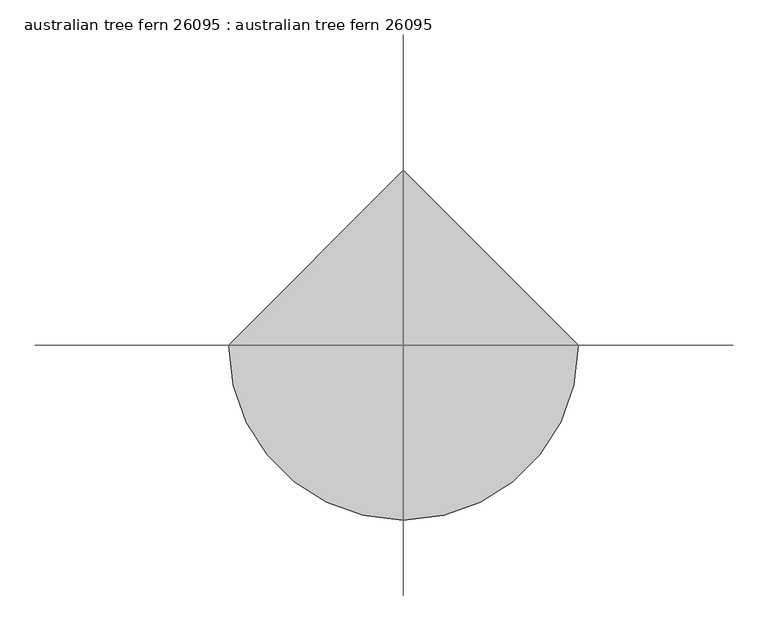
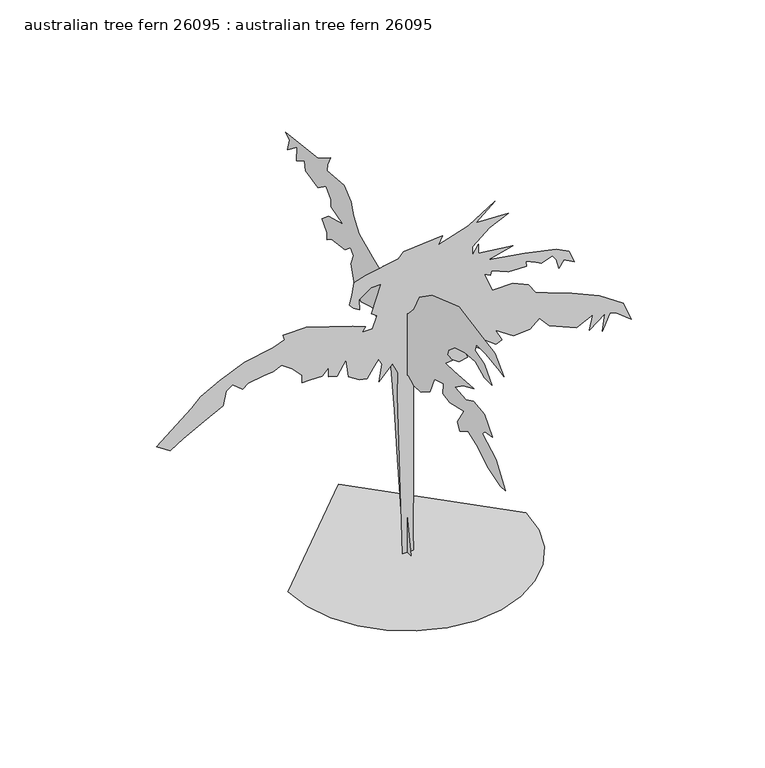
"""IFC4 building model written with IfcOpenShell, lengths in millimetres: proxy geometry, australian tree fern 26095 : australian tree fern 26095."""

from ifc_helpers import new_model, si_unit, origin, place, context, project, spatial, triangles, source, transform, mapped, element, save


def australian_tree_fern_26095_australian_tree_fern_26095_77f1a640(model_context):
    return source(origin(), model_context, "Body", "Tessellation", [
        triangles([(-639.0365753, 0.0, 0.0007159), (-622.1405136, -146.4247652, 0.0007159), (-574.0277527, -280.8912123, 0.0007159), (-498.5465315, -399.5499215, 0.0007159), (-399.5499215, -498.5465315, 0.0007159), (-280.8912123, -574.0277527, 0.0007159), (-146.4247652, -622.1405136, 0.0007159), (2.79e-05, -639.0365753, 0.0007159), (146.4247652, -622.1429844, 0.0007159), (280.8912123, -574.0277527, 0.0007159), (399.5499215, -498.5465315, 0.0007159), (498.5465315, -399.5499215, 0.0007159), (574.0277527, -280.8912123, 0.0007159), (622.1405136, -146.4247652, 0.0007159), (639.0365753, 5.59e-05, 0.0007159), (-8.38e-05, 639.0365753, 0.0007159), (470.2991641, -3.5e-05, 1828.8014534), (368.5593713, -2.98e-05, 1741.5955845), (542.9711454, -2.94e-05, 1734.3285862), (441.231389, -2.66e-05, 1687.0922253), (350.3907492, -2.2e-05, 1610.7880165), (350.3907492, -1.92e-05, 1563.5516556), (383.0932589, -2.22e-05, 1614.4202076), (383.0932589, -1.92e-05, 1563.5516556), (568.4067295, -1.79e-05, 1541.750806), (437.5966181, -1.59e-05, 1509.0482964), (633.8092781, -1.4e-05, 1476.3456413), (800.9540903, -1.18e-05, 1440.0109406), (869.9913008, -9.7e-06, 1403.673769), (899.0591486, -5.5e-06, 1334.6364132), (840.9235256, -7.5e-06, 1367.3389229), (815.4879416, -5.1e-06, 1327.3695602), (800.9540903, -8.4e-06, 1381.8729195), (779.1532408, -1.01e-05, 1410.9406219), (721.015147, -8.8e-06, 1389.1397724), (691.9473719, -9.7e-06, 1403.673769), (637.4440126, -1.12e-05, 1429.1092804), (641.0762037, -9.4e-06, 1400.0414326), (597.4745047, -9.4e-06, 1400.0414326), (542.9711454, -9.7e-06, 1403.673769), (452.1330491, -1.18e-05, 1440.0109406), (448.4983146, -1.03e-05, 1414.5754292), (415.7958049, -1.14e-05, 1432.7440876), (459.4000111, -5.1e-06, 1327.3695602), (568.4067295, -5.1e-06, 1327.3695602), (651.9778639, -2.9e-06, 1291.0347141), (688.3126373, 3e-07, 1236.5313549), (753.7176567, 1.8e-06, 1211.0958435), (884.5252247, 4.9e-06, 1160.2246754), (1033.5014511, 8.7e-06, 1094.8221268), (1160.6767553, 1.39e-05, 1007.6162579), (1204.2784544, 2.02e-05, 902.2417305), (1120.70732, 1.63e-05, 967.6468225), (1088.0048103, 1.59e-05, 974.9137482), (1048.0353024, 2.11e-05, 887.7078793), (1062.5692263, 1.55e-05, 982.1806738), (978.9980919, 1.94e-05, 916.7781979), (997.1666777, 1.44e-05, 1000.3493322), (909.9608088, 1.7e-05, 956.7450897), (764.6193169, 1.33e-05, 1018.5179907), (710.1159576, 9.6e-06, 1080.2882755), (659.2448622, 1.22e-05, 1036.684033), (572.0389206, 1.26e-05, 1029.4171074), (473.9338986, 8.7e-06, 1094.8221268), (510.2686357, 1.26e-05, 1029.4171074), (477.5660897, 1.35e-05, 1014.8831835), (324.9577085, 6.6e-06, 1131.1569002), (419.4305394, 1.44e-05, 1000.3493322), (284.9882369, 8.7e-06, 1094.8221268), (324.9577085, 1.48e-05, 993.0824066), (277.7212749, 1.52e-05, 985.8154083), (190.5151335, 1.16e-05, 1047.5857658), (88.7756132, 9.6e-06, 1080.2882755), (194.1488688, 1.52e-05, 985.8154083), (30.6385209, 1.11e-05, 1054.8526915), (34.2719928, 1.57e-05, 978.5484827), (34.2719928, 3.32e-05, 684.2282936), (34.2719928, 4.84e-05, 429.8801196), (30.6385209, 6.77e-05, 106.4923825), (34.2719928, 7.35e-05, 0.0013276), (-23.8650472, 7.39e-05, 0.0007003), (-52.9336422, 1.98e-05, 909.5111996), (-49.2999159, 1.22e-05, 1036.684033), (-78.3684632, 8.5e-06, 1098.4543905), (-151.0396997, 1.31e-05, 1022.1501818), (-136.5055487, 7.5e-06, 1116.6229763), (-154.6734259, 5.5e-06, 1149.325486), (-183.7417098, 7.9e-06, 1109.3560507), (-216.4437289, 1.07e-05, 1062.1196171), (-256.4132006, 1.03e-05, 1069.3865427), (-314.5512943, 8.1e-06, 1105.7213161), (-329.0852182, 2e-06, 1207.461109), (-376.3216155, 6.6e-06, 1131.1569002), (-423.5580491, 5.7e-06, 1145.6907515), (-423.5580491, 2.7e-06, 1196.5619196), (-456.2580153, 4.9e-06, 1160.2246754), (-518.0283365, 4.9e-06, 1160.2246754), (-565.2647701, 4.9e-06, 1160.2246754), (-565.2647701, 2.3e-06, 1203.8289179), (-619.7706728, -1e-06, 1258.3322044), (-674.2714886, -3.4e-06, 1298.3017124), (-721.5079222, -2.1e-06, 1276.5008629), (-772.3790903, -1.9e-06, 1272.866201), (-855.9502247, -1e-06, 1258.3322044), (-885.0205433, 3e-07, 1236.5313549), (-939.5239025, -2.3e-06, 1280.133054), (-972.2238688, -8e-07, 1254.6975426), (-990.3925272, 3.8e-06, 1178.3933338), (-1092.13232, 6.8e-06, 1127.5247091), (-1204.773773, 1.05e-05, 1065.7543516), (-1273.8110561, 1.31e-05, 1022.1501818), (-1346.4830738, 1.03e-05, 1069.3865427), (-1157.5373394, 1.2e-06, 1221.9975037), (-1110.3009058, -1.9e-06, 1272.866201), (-1008.561113, -5.1e-06, 1327.3695602), (-874.1188105, -8.6e-06, 1385.5075813), (-721.5079222, -1.03e-05, 1414.5754292), (-659.7375647, -1.16e-05, 1436.3762787), (-667.004563, -1.33e-05, 1465.4439812), (-539.8317295, -1.33e-05, 1465.4439812), (-416.2885437, -1.1e-05, 1425.4770893), (-292.7479377, -8.6e-06, 1385.5075813), (-223.7109271, -7.1e-06, 1360.0720699), (-241.8788043, -5.5e-06, 1334.6364132), (-187.3751907, -5.5e-06, 1334.6364132), (-161.9403697, -9.4e-06, 1400.0414326), (-191.0089079, -1.07e-05, 1421.8422821), (-140.1390206, -1.96e-05, 1570.8185085), (-194.6423889, -1.96e-05, 1570.8185085), (-260.0454098, -1.68e-05, 1523.5821476), (-256.4132006, -1.33e-05, 1465.4439812), (-289.1157284, -1.46e-05, 1487.2474468), (-310.9165598, -1.62e-05, 1512.6804874), (-296.3826722, -1.94e-05, 1567.1838467), (-285.4809939, -2.31e-05, 1628.956675), (-220.0774642, -2.44e-05, 1650.7575245), (-45.666444, -2.63e-05, 1683.4600342), (-20.2313959, -2.81e-05, 1712.5277367), (190.5151335, -2.92e-05, 1730.6963951), (168.7137935, -2.66e-05, 1687.0922253), (328.5898996, -2.96e-05, 1737.9633934), (3.03e-05, -861.8582216, 1549.8330162), (2.4e-05, -733.5424347, 1570.5289913), (2.01e-05, -646.6209961, 1570.5289913), (2.06e-05, -630.0627771, 1529.1370411), (2.54e-05, -721.12437, 1504.3009117), (3.07e-05, -787.3523769, 1425.6574562), (2.76e-05, -716.9866865, 1425.6574562), (2.26e-05, -634.2029314, 1467.0492611), (1.86e-05, -539.0011479, 1458.7689526), (1.52e-05, -443.8018716, 1429.7951397), (1.41e-05, -385.8542459, 1380.1253517), (1.46e-05, -373.4361812, 1347.0113846), (1.68e-05, -423.1059328, 1347.0113846), (1.55e-05, -356.8778895, 1289.0637589), (1.89e-05, -435.5239975, 1293.2039131), (2.69e-05, -621.7848667, 1305.6220505), (2.36e-05, -518.3052092, 1260.089946), (2.19e-05, -443.8018716, 1206.2800037), (2.68e-05, -547.2815291, 1198.0020933), (2.89e-05, -617.6471832, 1231.1161331), (3.37e-05, -716.9866865, 1218.6980684), (3.97e-05, -795.6302147, 1135.9143133), (3.69e-05, -725.2645243, 1123.4987921), (3.66e-05, -700.4309383, 1098.6626627), (4.42e-05, -824.6040276, 1028.2969723), (5.2e-05, -915.6656204, 904.1213396), (4.99e-05, -865.9959051, 899.9836561), (4.34e-05, -745.9604994, 937.2353794), (3.69e-05, -642.4808418, 999.3231594), (3.26e-05, -567.9774679, 1032.4371992), (3.06e-05, -489.3313963, 982.7648678), (2.84e-05, -468.6354575, 1024.1567453), (2.82e-05, -530.7232738, 1123.4987921), (2.33e-05, -398.2697671, 1090.3847523), (2e-05, -332.0443036, 1102.802817), (1.84e-05, -336.1819871, 1160.7504427), (1.55e-05, -253.3997399, 1135.9143133), (1.65e-05, -212.0081348, 1040.715037), (1.44e-05, -129.2246341, 986.9050947), (1.15e-05, -62.9981487, 982.7648678), (8.4e-06, -13.3280768, 1011.7412241), (6.8e-06, 32.2026538, 999.3231594), (4.5e-06, 52.8985925, 1044.8527205), (4.9e-06, 81.8726461, 986.9050947), (7e-06, 86.0118375, 912.3991774), (1.57e-05, 57.0377794, 664.0505281), (2.77e-05, 19.7852431, 316.3597959), (3.93e-05, -34.0238362, 0.0007149), (3.64e-05, 36.3418406, 0.0), (3.07e-05, 52.8985925, 167.3503229), (1.97e-05, 90.1512742, 477.7870791), (1.08e-05, 119.1250779, 734.4162186), (1.5e-06, 156.3777732, 991.0453217), (-4.8e-06, 210.1869524, 1119.3585651), (-7.3e-06, 268.135323, 1119.3585651), (-1.14e-05, 305.3869918, 1198.0020933), (-1.38e-05, 371.6149987, 1181.4464178), (-1.58e-05, 429.5625881, 1160.7504427), (-2.04e-05, 491.6504045, 1222.8382954), (-2.47e-05, 520.6242173, 1322.177726), (-2.55e-05, 499.9282785, 1380.1253517), (-2.76e-05, 528.9020914, 1409.0991646), (-2.86e-05, 578.5718067, 1367.7072144), (-3.37e-05, 702.7474394, 1351.1515388), (-3.47e-05, 744.1393169, 1322.177726), (-3.59e-05, 744.1393169, 1363.5696762), (-3.96e-05, 793.8090322, 1413.2393188), (-3.83e-05, 731.7212523, 1462.9091068), (-3.35e-05, 599.2677455, 1500.1607574), (-3.93e-05, 706.8876663, 1533.2747246), (-4.06e-05, 711.0252771, 1570.5289913), (-4.41e-05, 756.5573816, 1620.1987793), (-4.58e-05, 831.0607555, 1566.3888371), (-5.18e-05, 946.9584778, 1591.2223503), (-5.36e-05, 955.2363155, 1640.8946091), (-5.57e-05, 1029.7422329, 1599.5028042), (-5.79e-05, 1025.602006, 1678.1462597), (-5.98e-05, 1112.525988, 1611.9183254), (-6.09e-05, 1095.9676964, 1674.0061054), (-6.33e-05, 1133.2218904, 1698.8422348), (-5.08e-05, 831.0607555, 1731.9562019), (-4.78e-05, 715.1655041, 1806.4596485), (-4.73e-05, 739.99909, 1752.652177), (-4.64e-05, 748.2795439, 1711.2603722), (-3.97e-05, 586.8496808, 1727.8160477), (-3.52e-05, 520.6242173, 1674.0061054), (-3.23e-05, 499.9282785, 1607.7806419), (-2.78e-05, 446.1183363, 1537.4150242), (-2.05e-05, 321.9452471, 1479.4647823), (-1.04e-05, 143.960199, 1409.0991646), (-1.65e-05, 226.7434454, 1487.7452362), (-9.7e-06, 114.9858956, 1429.7951397), (-2.2e-06, -0.9105653, 1351.1515388), (-1.4e-06, -62.9981487, 1417.3796185), (-2.2e-06, -112.668141, 1516.7190491), (7e-07, -232.7038011, 1599.5028042), (9.2e-06, -481.0535222, 1686.4242428), (2.03e-05, -700.4309383, 1645.0322926), (2.61e-05, -816.3261898, 1624.3363174), (3.23e-05, -899.1099449, 1541.5525623)], [[15, 16, 1], [14, 15, 1], [14, 1, 2], [13, 14, 2], [13, 2, 3], [13, 3, 4], [12, 13, 4], [11, 12, 4], [11, 4, 5], [11, 5, 6], [11, 6, 7], [11, 7, 8], [11, 8, 9], [11, 9, 10], [141, 17, 18], [54, 55, 56], [73, 74, 75], [67, 68, 69], [24, 25, 26], [18, 19, 20], [51, 52, 53], [22, 23, 24], [84, 85, 86], [29, 30, 31], [56, 57, 58], [31, 32, 33], [130, 131, 132], [138, 139, 140], [41, 42, 43], [111, 112, 113], [110, 111, 113], [109, 110, 113], [122, 123, 124], [118, 119, 120], [18, 20, 21], [141, 18, 21], [69, 70, 71], [69, 71, 72], [28, 29, 31], [28, 31, 33], [28, 33, 34], [27, 28, 34], [27, 34, 35], [27, 35, 36], [27, 36, 37], [130, 132, 133], [130, 133, 134], [50, 51, 53], [50, 53, 54], [50, 54, 56], [50, 56, 58], [140, 141, 21], [37, 38, 39], [64, 65, 66], [64, 66, 67], [80, 81, 82], [79, 80, 82], [78, 79, 82], [77, 78, 82], [76, 77, 82], [76, 82, 83], [75, 76, 83], [97, 98, 99], [49, 50, 58], [49, 58, 59], [49, 59, 60], [48, 49, 60], [48, 60, 61], [47, 48, 61], [129, 130, 134], [129, 134, 135], [129, 135, 136], [129, 136, 137], [128, 129, 137], [108, 109, 113], [108, 113, 114], [107, 108, 114], [107, 114, 115], [106, 107, 115], [106, 115, 116], [105, 106, 116], [104, 105, 116], [103, 104, 116], [103, 116, 117], [102, 103, 117], [101, 102, 117], [101, 117, 118], [75, 83, 84], [26, 27, 37], [26, 37, 39], [26, 39, 40], [26, 40, 41], [26, 41, 43], [92, 93, 94], [92, 94, 95], [126, 127, 128], [101, 118, 120], [100, 101, 120], [100, 120, 121], [99, 100, 121], [97, 99, 121], [96, 97, 121], [95, 96, 121], [95, 121, 122], [92, 95, 122], [92, 122, 124], [140, 21, 22], [88, 89, 90], [24, 26, 43], [22, 24, 43], [88, 90, 91], [88, 91, 92], [88, 92, 124], [87, 88, 124], [87, 124, 125], [47, 61, 62], [47, 62, 63], [47, 63, 64], [46, 47, 64], [45, 46, 64], [44, 45, 64], [44, 64, 67], [43, 44, 67], [137, 138, 140], [128, 137, 140], [126, 128, 140], [126, 140, 22], [126, 22, 43], [126, 43, 67], [126, 67, 69], [126, 69, 72], [126, 72, 73], [125, 126, 73], [87, 125, 73], [87, 73, 75], [87, 75, 84], [87, 84, 86], [231, 232, 233], [156, 157, 158], [240, 241, 142], [222, 223, 224], [218, 219, 220], [220, 221, 222], [218, 220, 222], [153, 154, 155], [240, 142, 143], [239, 240, 143], [146, 147, 148], [205, 206, 207], [162, 163, 164], [156, 158, 159], [216, 217, 218], [216, 218, 222], [166, 167, 168], [166, 168, 169], [222, 224, 225], [239, 143, 144], [238, 239, 144], [146, 148, 149], [145, 146, 149], [165, 166, 169], [165, 169, 170], [207, 208, 209], [188, 189, 190], [188, 190, 191], [188, 191, 192], [187, 188, 192], [187, 192, 193], [186, 187, 193], [186, 193, 194], [185, 186, 194], [171, 172, 173], [171, 173, 174], [145, 149, 150], [155, 156, 159], [165, 170, 171], [165, 171, 174], [175, 176, 177], [182, 183, 184], [205, 207, 209], [205, 209, 210], [204, 205, 210], [203, 204, 210], [161, 162, 164], [161, 164, 165], [161, 165, 174], [160, 161, 174], [159, 160, 174], [159, 174, 175], [159, 175, 177], [155, 159, 177], [238, 144, 145], [238, 145, 150], [237, 238, 150], [237, 150, 151], [237, 151, 152], [236, 237, 152], [235, 236, 152], [235, 152, 153], [235, 153, 155], [235, 155, 177], [235, 177, 178], [234, 235, 178], [234, 178, 179], [234, 179, 180], [234, 180, 181], [234, 181, 182], [234, 182, 184], [231, 233, 234], [231, 234, 184], [214, 215, 216], [214, 216, 222], [213, 214, 222], [213, 222, 225], [213, 225, 226], [212, 213, 226], [212, 226, 227], [212, 227, 228], [211, 212, 228], [210, 211, 228], [210, 228, 229], [203, 210, 229], [203, 229, 230], [202, 203, 230], [184, 185, 194], [184, 194, 195], [231, 184, 195], [230, 231, 195], [230, 195, 196], [230, 196, 197], [202, 230, 197], [202, 197, 198], [201, 202, 198], [200, 201, 198], [199, 200, 198]], closed=False),
    ])


if __name__ == "__main__":
    model = new_model("IFC4")
    model_context = context("Model", 3, world=origin())
    ifc_project = project(units=[si_unit("LENGTHUNIT", "METRE", prefix="MILLI")], contexts=[model_context])
    site = spatial("IfcSite", under=ifc_project)
    building = spatial("IfcBuilding", under=site)
    placement = place(None, origin())
    australian_tree_fern_26095_australian_tree_fern_26095_shape = australian_tree_fern_26095_australian_tree_fern_26095_77f1a640(model_context)
    element("IfcBuildingElementProxy", 1, Name="australian tree fern 26095 : australian tree fern 26095", ObjectType="australian tree fern 26095 : australian tree fern 26095", at=placement, inside=building, context=model_context, shape_type="MappedRepresentation", body=[
        mapped(australian_tree_fern_26095_australian_tree_fern_26095_shape, transform((0.0, 0.0, 0.0), x_axis=(1.0, 0.0, 0.0), y_axis=(0.0, 1.0, 0.0), z_axis=(0.0, 0.0, 1.0))),
    ])
    save(model, "model.ifc")

# Revit data of these elements
# Type "australian tree fern 26095 : australian tree fern 26095"
#   built-in parameter 1005195 = "RPC-16-FVCN-UWG0-AP53-A000-ST1L-LVER-AU"
#   Height = 0
